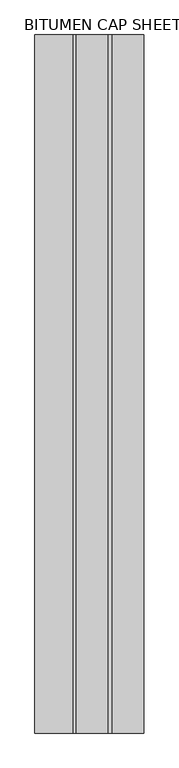
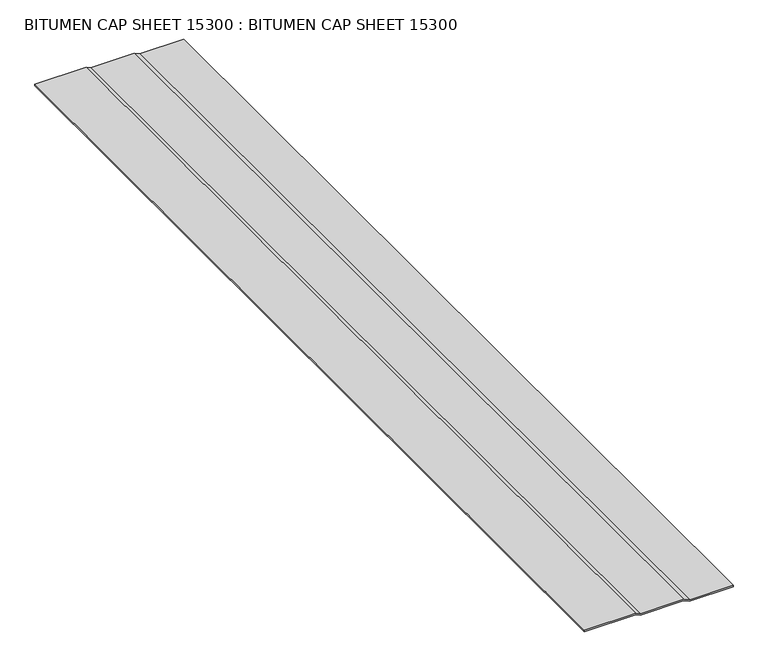
"""IFC4 building model written with IfcOpenShell, lengths in millimetres: proxy geometry, BITUMEN CAP SHEET 15300 : BITUMEN CAP SHEET 15300."""

from ifc_helpers import new_model, si_unit, frame, origin, place, context, project, spatial, polyline, outline, extrude, source, transform, mapped, element, save


def bitumen_cap_sheet_15300_bitumen_cap_sheet_15300_313e2dc3(model_context):
    return source(origin(), model_context, "Body", "SweptSolid", [
        extrude(outline(polyline([(40259.2002678, -2469.2761954), (40262.3752678, -2469.2761954), (40262.3752678, -2560.795457), (40267.6612773, -2573.2602756), (40267.6612773, -2663.9440313), (40271.9940719, -2673.6609328), (40271.9940719, -2781.5474293), (40268.8188423, -2781.5474293), (40268.8188423, -2674.3362183), (40264.4862773, -2664.6198318), (40264.4862773, -2573.9056756), (40259.2002678, -2561.440857), (40259.2002678, -2469.2761954)])), frame((0.0, -1052.8906574, 0.0), z_axis=(0.0, 1.0, 0.0), x_axis=(0.0, 0.0, 1.0)), (0.0, 0.0, 1.0), 2000.25),
    ])


if __name__ == "__main__":
    model = new_model("IFC4")
    model_context = context("Model", 3, world=origin())
    ifc_project = project(units=[si_unit("LENGTHUNIT", "METRE", prefix="MILLI")], contexts=[model_context])
    site = spatial("IfcSite", under=ifc_project)
    building = spatial("IfcBuilding", under=site)
    placement = place(None, origin())
    bitumen_cap_sheet_15300_bitumen_cap_sheet_15300_shape = bitumen_cap_sheet_15300_bitumen_cap_sheet_15300_313e2dc3(model_context)
    element("IfcBuildingElementProxy", 1, Name="BITUMEN CAP SHEET 15300 : BITUMEN CAP SHEET 15300", ObjectType="BITUMEN CAP SHEET 15300 : BITUMEN CAP SHEET 15300", at=placement, inside=building, context=model_context, shape_type="MappedRepresentation", body=[
        mapped(bitumen_cap_sheet_15300_bitumen_cap_sheet_15300_shape, transform((0.0, 0.0, 0.0), x_axis=(1.0, 0.0, 0.0), y_axis=(0.0, 1.0, 0.0), z_axis=(0.0, 0.0, 1.0))),
    ])
    save(model, "model.ifc")

# Revit data of these elements
# Type "BITUMEN CAP SHEET 15300 : BITUMEN CAP SHEET 15300"
#   NameOverride = "BITUMEN CAP SHEET"
# Element 1 (IfcBuildingElementProxy, "BITUMEN CAP SHEET 15300 : BITUMEN CAP SHEET 15300")
#   Materials on its faces: "MODIFIED BITUMEN GRANULE SURFACED CAP SHEET"
# Materials
#   "MODIFIED BITUMEN GRANULE SURFACED CAP SHEET": class "Unassigned", colour RGB 85 85 127, transparency 0
